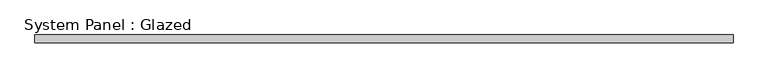
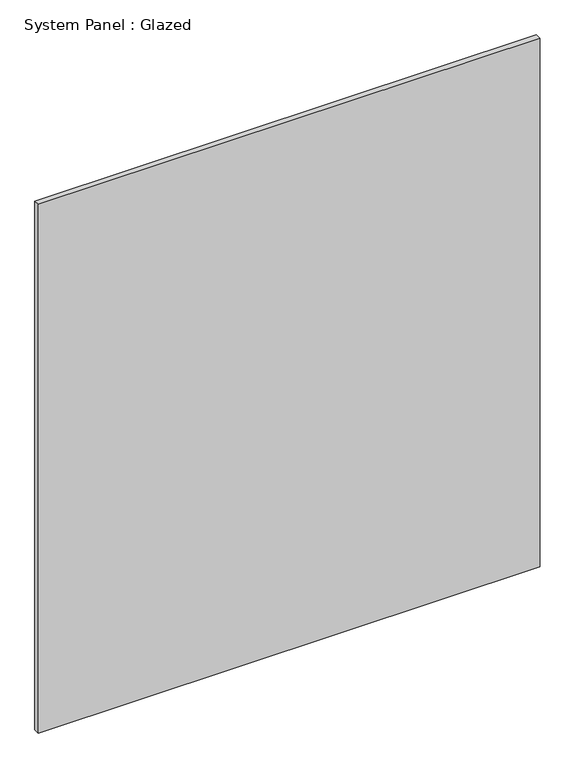
"""IFC4 building model written with IfcOpenShell, lengths in millimetres: plate geometry, System Panel : Glazed."""

from ifc_helpers import new_model, si_unit, origin, origin_with_axes, place, context, project, spatial, polyline, outline, extrude, source, transform, mapped, element, save


def system_panel_glazed_bdc57ba0(model_context):
    return source(origin(), model_context, "Body", "SweptSolid", [
        extrude(outline(polyline([(1087.5, 24.5), (-1087.5, 24.5), (-1087.5, 49.5), (1087.5, 49.5), (1087.5, 24.5)])), origin_with_axes(), (0.0, 0.0, 1.0), 2422.0381538),
    ])


if __name__ == "__main__":
    model = new_model("IFC4")
    model_context = context("Model", 3, world=origin())
    ifc_project = project(units=[si_unit("LENGTHUNIT", "METRE", prefix="MILLI")], contexts=[model_context])
    site = spatial("IfcSite", under=ifc_project)
    building = spatial("IfcBuilding", under=site)
    placement = place(None, origin())
    system_panel_glazed_shape = system_panel_glazed_bdc57ba0(model_context)
    element("IfcPlate", 1, ObjectType="System Panel : Glazed", at=placement, inside=building, context=model_context, shape_type="MappedRepresentation", body=[
        mapped(system_panel_glazed_shape, transform((0.0, 0.0, 0.0), x_axis=(1.0, 0.0, 0.0), y_axis=(0.0, 1.0, 0.0), z_axis=(0.0, 0.0, 1.0))),
    ])
    save(model, "model.ifc")

# Revit data of these elements
# Type "System Panel : Glazed"
#   Keynote = "H11"
#   Construction Type Id = "GSP4R"
#   Analytic Construction = "1/8 in Pilkington single glazing"
#   Visual Light Transmittance = 0.9
#   Solar Heat Gain Coefficient = 0.86
#   Heat Transfer Coefficient (U) = 6.7069 W/(m²·K)
#   Define Thermal Properties by = 1
# Element 1 (IfcPlate, "System Panel : Glazed")
#   Materials on its faces: "Glass"
# Materials
#   "Glass": class "Glass", colour RGB 0 128 192, transparency 0.9, Description = "Soda Lime Glass", Cost = 0
